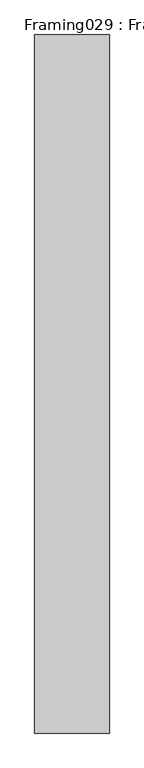
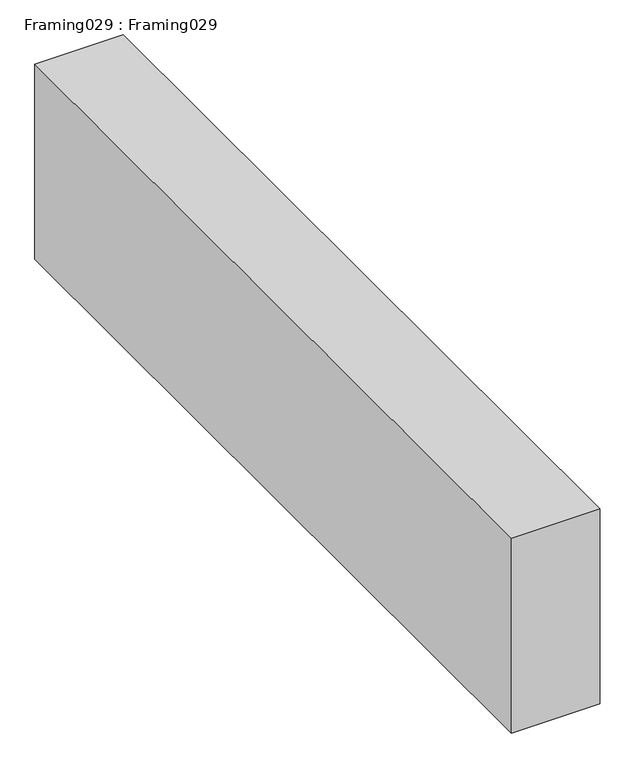
"""IFC4 building model written with IfcOpenShell, lengths in millimetres: proxy geometry, Framing029 : Framing029."""

from ifc_helpers import new_model, si_unit, frame, origin, place, context, project, spatial, polyline, outline, extrude, source, transform, mapped, element, save


def framing029_framing029_90286849(model_context):
    return source(origin(), model_context, "Body", "SweptSolid", [
        extrude(outline(polyline([(12687.8178845, -2827.7925368), (12687.8178845, -4253.3675368), (12535.4178845, -4253.3675368), (12535.4178845, -2827.7925368), (12687.8178845, -2827.7925368)])), frame((0.0, 0.0, 39757.096), z_axis=(0.0, 0.0, 1.0), x_axis=(1.0, 0.0, 0.0)), (0.0, 0.0, 1.0), 355.6),
    ])


if __name__ == "__main__":
    model = new_model("IFC4")
    model_context = context("Model", 3, world=origin())
    ifc_project = project(units=[si_unit("LENGTHUNIT", "METRE", prefix="MILLI")], contexts=[model_context])
    site = spatial("IfcSite", under=ifc_project)
    building = spatial("IfcBuilding", under=site)
    placement = place(None, origin())
    framing029_framing029_shape = framing029_framing029_90286849(model_context)
    element("IfcBuildingElementProxy", 1, Name="Framing029 : Framing029", ObjectType="Framing029 : Framing029", at=placement, inside=building, context=model_context, shape_type="MappedRepresentation", body=[
        mapped(framing029_framing029_shape, transform((0.0, 0.0, 0.0), x_axis=(1.0, 0.0, 0.0), y_axis=(0.0, 1.0, 0.0), z_axis=(0.0, 0.0, 1.0))),
    ])
    save(model, "model.ifc")

# Revit data of these elements
# Type "Framing029 : Framing029"
#   NameOverride = "Framing029"
# Element 1 (IfcBuildingElementProxy, "Framing029 : Framing029")
#   Materials on its faces: "WOOD FRAMING (SEE STRUCT DWGS)"
# Materials
#   "WOOD FRAMING (SEE STRUCT DWGS)": class "Unassigned", colour RGB 224 188 168, transparency 0, Cost = 0
